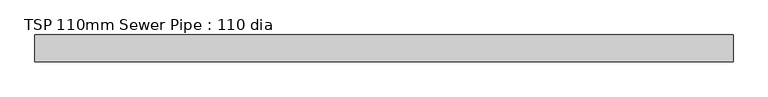
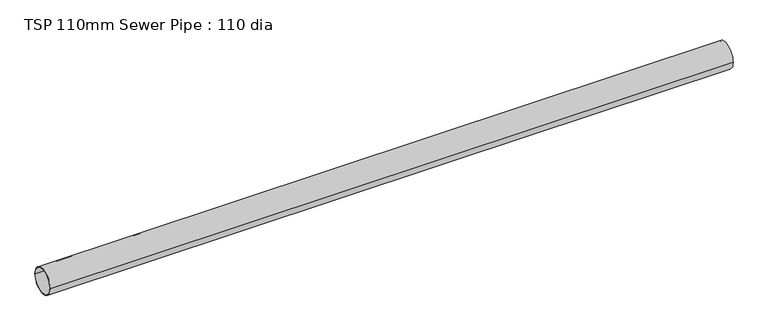
"""IFC4 building model written with IfcOpenShell, lengths in millimetres: flow terminal geometry, TSP 110mm Sewer Pipe : 110 dia."""

from ifc_helpers import new_model, si_unit, point, frame, origin, origin_2d, place, context, project, spatial, circle_curve, trimmed, segment, composite_curve, outline, extrude, source, transform, mapped, element, save


def tsp_110mm_sewer_pipe_110_dia_48d26cdf(model_context):
    return source(origin(), model_context, "Body", "SweptSolid", [
        extrude(outline(composite_curve([segment(trimmed(circle_curve(origin_2d(), 55.0), [point((-55.0, 0.0))], [point((55.0, 0.0))], False, "CARTESIAN"), True, "CONTINUOUS"), segment(trimmed(circle_curve(origin_2d(), 55.0), [point((55.0, 0.0))], [point((-55.0, 0.0))], False, "CARTESIAN"), True, "CONTINUOUS")], self_intersect=False), holes=[composite_curve([segment(trimmed(circle_curve(origin_2d(), 52.0), [point((-52.0, 0.0))], [point((52.0, 0.0))], True, "CARTESIAN"), True, "CONTINUOUS"), segment(trimmed(circle_curve(origin_2d(), 52.0), [point((52.0, 0.0))], [point((-52.0, 0.0))], True, "CARTESIAN"), True, "CONTINUOUS")], self_intersect=False)]), frame((0.0, 0.0, 0.0), z_axis=(1.0, 0.0, 0.0), x_axis=(0.0, 1.0, 0.0)), (0.0, 0.0, 1.0), 2867.3179977),
    ])


if __name__ == "__main__":
    model = new_model("IFC4")
    model_context = context("Model", 3, world=origin())
    ifc_project = project(units=[si_unit("LENGTHUNIT", "METRE", prefix="MILLI")], contexts=[model_context])
    site = spatial("IfcSite", under=ifc_project)
    building = spatial("IfcBuilding", under=site)
    placement = place(None, origin())
    tsp_110mm_sewer_pipe_110_dia_shape = tsp_110mm_sewer_pipe_110_dia_48d26cdf(model_context)
    element("IfcFlowTerminal", 1, ObjectType="TSP 110mm Sewer Pipe : 110 dia", at=placement, inside=building, context=model_context, shape_type="MappedRepresentation", body=[
        mapped(tsp_110mm_sewer_pipe_110_dia_shape, transform((0.0, 0.0, 0.0), x_axis=(1.0, 0.0, 0.0), y_axis=(0.0, 1.0, 0.0), z_axis=(0.0, 0.0, 1.0))),
    ])
    save(model, "model.ifc")

# Revit data of these elements
# Type "TSP 110mm Sewer Pipe : 110 dia"
#   Model = "TSP_110SWB"
#   Model = "TSP_110SWB"
#   Pipe length [instance default] = 1200 mm
#   Pipe dia = 110 mm
#   built-in parameter 1001306 [instance default] = 3.93701 (stored number, unit not read)
#   Default Elevation = 0
# Element 1 (IfcFlowTerminal, "TSP 110mm Sewer Pipe : 110 dia")
#   Pipe length = 2867.318 mm
#   built-in parameter 1001306 = 9.40721 (stored number, unit not read)
#   Materials on its faces: "Laminate, Brown, Matte"
# Materials
#   "Laminate, Brown, Matte": class "Plastic", colour RGB 128 64 0, transparency 0, Description = "Plastic Laminate - Red, Matte", Cost = 0
